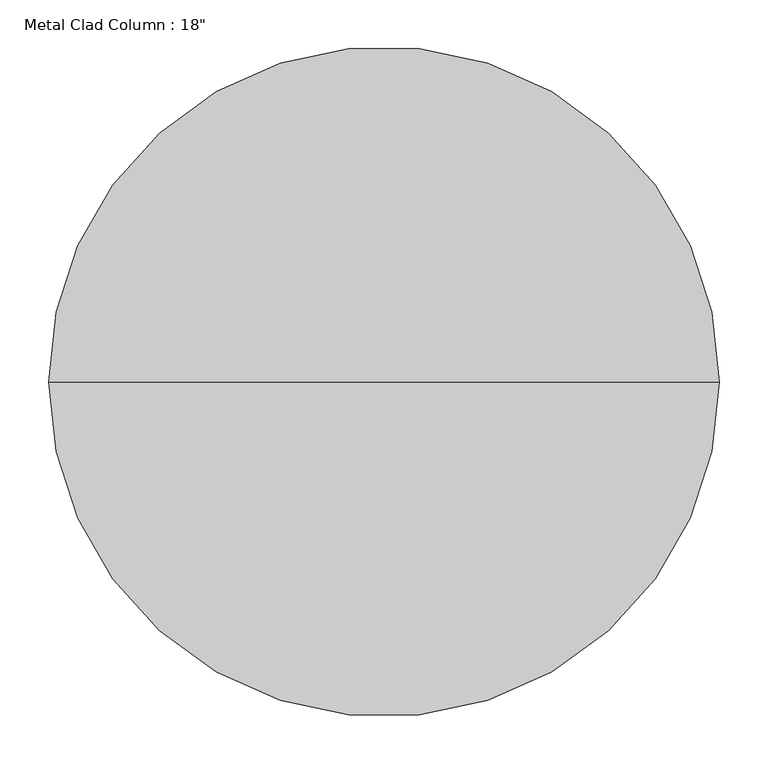
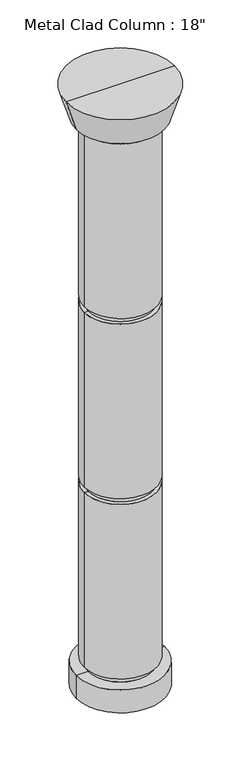
"""IFC4 building model written with IfcOpenShell, lengths in millimetres: column geometry."""

from ifc_helpers import new_model, si_unit, frame, origin, place, context, project, spatial, polyline, circle_curve, source, transform, mapped, element, save
from ifc_brep_helpers import plane_surface, cylinder_surface, revolved_surface, advanced_brep


def column_c029851a(model_context):
    return source(origin(), model_context, "Body", "AdvancedBrep", [
        advanced_brep(
        [(0.0, 0.0, 0.0), (-279.4, 0.0, 0.0), (279.4, 0.0, 0.0), (-279.4, 0.0, 152.4), (279.4, 0.0, 152.4), (203.2, 0.0, 1392.6), (-203.2, 0.0, 1392.6), (-228.6, 0.0, 1392.6), (228.6, 0.0, 1392.6), (-228.6, 0.0, 2556.6), (228.6, 0.0, 2556.6), (203.2, 0.0, 1354.5), (-203.2, 0.0, 1354.5), (228.6, 0.0, 1354.5), (-228.6, 0.0, 1354.5), (228.6, 0.0, 190.5), (-228.6, 0.0, 190.5), (203.2, 0.0, 190.5), (-203.2, 0.0, 190.5), (203.2, 0.0, 152.4), (-203.2, 0.0, 152.4), (279.4, 0.0, 3796.8), (-279.4, 0.0, 3796.8), (-342.9, 0.0, 4000.0), (342.9, 0.0, 4000.0), (0.0, 0.0, 4000.0), (203.2, 0.0, 3796.8), (-203.2, 0.0, 3796.8), (203.2, 0.0, 3758.7), (-203.2, 0.0, 3758.7), (228.6, 0.0, 3758.7), (-228.6, 0.0, 3758.7), (228.6, 0.0, 2594.7), (-228.6, 0.0, 2594.7), (203.2, 0.0, 2594.7), (-203.2, 0.0, 2594.7), (203.2, 0.0, 2556.6), (-203.2, 0.0, 2556.6)],
        [
            (0, 1),
            (1, 2, circle_curve(frame((0.0, 0.0, 0.0), z_axis=(0.0, 0.0, -1.0), x_axis=(-1.0, 0.0, 0.0)), 279.4)),
            (2, 0),
            (2, 1, circle_curve(frame((0.0, 0.0, 0.0), z_axis=(0.0, 0.0, -1.0), x_axis=(-1.0, 0.0, 0.0)), 279.4)),
            (1, 3),
            (3, 4, circle_curve(frame((0.0, 0.0, 152.4), z_axis=(0.0, 0.0, -1.0), x_axis=(-1.0, 0.0, 0.0)), 279.4)),
            (4, 2),
            (4, 3, circle_curve(frame((0.0, 0.0, 152.4), z_axis=(0.0, 0.0, -1.0), x_axis=(-1.0, 0.0, 0.0)), 279.4)),
            (5, 6, circle_curve(frame((0.0, 0.0, 1392.6), z_axis=(0.0, 0.0, 1.0), x_axis=(-1.0, 0.0, 0.0)), 203.2)),
            (6, 7),
            (7, 8, circle_curve(frame((0.0, 0.0, 1392.6), z_axis=(0.0, 0.0, -1.0), x_axis=(-1.0, 0.0, 0.0)), 228.6)),
            (8, 5),
            (7, 9),
            (9, 10, circle_curve(frame((0.0, 0.0, 2556.6), z_axis=(0.0, 0.0, -1.0), x_axis=(-1.0, 0.0, 0.0)), 228.6)),
            (10, 8),
            (7, 8, circle_curve(frame((0.0, 0.0, 1392.6), z_axis=(0.0, 0.0, 1.0), x_axis=(-1.0, 0.0, 0.0)), 228.6)),
            (10, 9, circle_curve(frame((0.0, 0.0, 2556.6), z_axis=(0.0, 0.0, -1.0), x_axis=(-1.0, 0.0, 0.0)), 228.6)),
            (6, 5, circle_curve(frame((0.0, 0.0, 1392.6), z_axis=(0.0, 0.0, 1.0), x_axis=(-1.0, 0.0, 0.0)), 203.2)),
            (11, 12, circle_curve(frame((0.0, 0.0, 1354.5), z_axis=(0.0, 0.0, 1.0), x_axis=(-1.0, 0.0, 0.0)), 203.2)),
            (12, 6),
            (5, 11),
            (12, 11, circle_curve(frame((0.0, 0.0, 1354.5), z_axis=(0.0, 0.0, 1.0), x_axis=(-1.0, 0.0, 0.0)), 203.2)),
            (13, 14, circle_curve(frame((0.0, 0.0, 1354.5), z_axis=(0.0, 0.0, 1.0), x_axis=(-1.0, 0.0, 0.0)), 228.6)),
            (14, 12),
            (11, 13),
            (14, 13, circle_curve(frame((0.0, 0.0, 1354.5), z_axis=(0.0, 0.0, 1.0), x_axis=(-1.0, 0.0, 0.0)), 228.6)),
            (15, 16, circle_curve(frame((0.0, 0.0, 190.5), z_axis=(0.0, 0.0, 1.0), x_axis=(-1.0, 0.0, 0.0)), 228.6)),
            (16, 14),
            (13, 15),
            (16, 15, circle_curve(frame((0.0, 0.0, 190.5), z_axis=(0.0, 0.0, 1.0), x_axis=(-1.0, 0.0, 0.0)), 228.6)),
            (17, 18, circle_curve(frame((0.0, 0.0, 190.5), z_axis=(0.0, 0.0, 1.0), x_axis=(-1.0, 0.0, 0.0)), 203.2)),
            (18, 16),
            (15, 17),
            (18, 17, circle_curve(frame((0.0, 0.0, 190.5), z_axis=(0.0, 0.0, 1.0), x_axis=(-1.0, 0.0, 0.0)), 203.2)),
            (19, 20, circle_curve(frame((0.0, 0.0, 152.4), z_axis=(0.0, 0.0, 1.0), x_axis=(-1.0, 0.0, 0.0)), 203.2)),
            (20, 18),
            (17, 19),
            (20, 19, circle_curve(frame((0.0, 0.0, 152.4), z_axis=(0.0, 0.0, 1.0), x_axis=(-1.0, 0.0, 0.0)), 203.2)),
            (3, 20),
            (19, 4),
            (21, 22, circle_curve(frame((0.0, 0.0, 3796.8), z_axis=(0.0, 0.0, 1.0), x_axis=(-1.0, 0.0, 0.0)), 279.4)),
            (22, 23),
            (23, 24, circle_curve(frame((0.0, 0.0, 4000.0), z_axis=(0.0, 0.0, -1.0), x_axis=(-1.0, 0.0, 0.0)), 342.9)),
            (24, 21),
            (23, 25),
            (25, 24),
            (23, 24, circle_curve(frame((0.0, 0.0, 4000.0), z_axis=(0.0, 0.0, 1.0), x_axis=(-1.0, 0.0, 0.0)), 342.9)),
            (22, 21, circle_curve(frame((0.0, 0.0, 3796.8), z_axis=(0.0, 0.0, 1.0), x_axis=(-1.0, 0.0, 0.0)), 279.4)),
            (26, 27, circle_curve(frame((0.0, 0.0, 3796.8), z_axis=(0.0, 0.0, 1.0), x_axis=(-1.0, 0.0, 0.0)), 203.2)),
            (27, 22),
            (21, 26),
            (27, 26, circle_curve(frame((0.0, 0.0, 3796.8), z_axis=(0.0, 0.0, 1.0), x_axis=(-1.0, 0.0, 0.0)), 203.2)),
            (28, 29, circle_curve(frame((0.0, 0.0, 3758.7), z_axis=(0.0, 0.0, 1.0), x_axis=(-1.0, 0.0, 0.0)), 203.2)),
            (29, 27),
            (26, 28),
            (29, 28, circle_curve(frame((0.0, 0.0, 3758.7), z_axis=(0.0, 0.0, 1.0), x_axis=(-1.0, 0.0, 0.0)), 203.2)),
            (30, 31, circle_curve(frame((0.0, 0.0, 3758.7), z_axis=(0.0, 0.0, 1.0), x_axis=(-1.0, 0.0, 0.0)), 228.6)),
            (31, 29),
            (28, 30),
            (31, 30, circle_curve(frame((0.0, 0.0, 3758.7), z_axis=(0.0, 0.0, 1.0), x_axis=(-1.0, 0.0, 0.0)), 228.6)),
            (32, 33, circle_curve(frame((0.0, 0.0, 2594.7), z_axis=(0.0, 0.0, 1.0), x_axis=(-1.0, 0.0, 0.0)), 228.6)),
            (33, 31),
            (30, 32),
            (33, 32, circle_curve(frame((0.0, 0.0, 2594.7), z_axis=(0.0, 0.0, 1.0), x_axis=(-1.0, 0.0, 0.0)), 228.6)),
            (34, 35, circle_curve(frame((0.0, 0.0, 2594.7), z_axis=(0.0, 0.0, 1.0), x_axis=(-1.0, 0.0, 0.0)), 203.2)),
            (35, 33),
            (32, 34),
            (35, 34, circle_curve(frame((0.0, 0.0, 2594.7), z_axis=(0.0, 0.0, 1.0), x_axis=(-1.0, 0.0, 0.0)), 203.2)),
            (36, 37, circle_curve(frame((0.0, 0.0, 2556.6), z_axis=(0.0, 0.0, 1.0), x_axis=(-1.0, 0.0, 0.0)), 203.2)),
            (37, 35),
            (34, 36),
            (37, 36, circle_curve(frame((0.0, 0.0, 2556.6), z_axis=(0.0, 0.0, 1.0), x_axis=(-1.0, 0.0, 0.0)), 203.2)),
            (9, 37),
            (36, 10),
        ],
        [
            plane_surface(frame((0.0, 0.0, 0.0), z_axis=(0.0, 0.0, -1.0), x_axis=(-1.0, 0.0, 0.0))),
            cylinder_surface(frame((0.0, 0.0, 4000.0), z_axis=(0.0, 0.0, -1.0), x_axis=(-1.0, 0.0, 0.0)), 279.4),
            plane_surface(frame((0.0, 0.0, 1392.6), z_axis=(0.0, 0.0, -1.0), x_axis=(-1.0, 0.0, 0.0))),
            cylinder_surface(frame((0.0, 0.0, 4000.0), z_axis=(0.0, 0.0, -1.0), x_axis=(-1.0, 0.0, 0.0)), 228.6),
            cylinder_surface(frame((0.0, 0.0, 4000.0), z_axis=(0.0, 0.0, -1.0), x_axis=(-1.0, 0.0, 0.0)), 203.2),
            plane_surface(frame((0.0, 0.0, 1354.5), z_axis=(0.0, 0.0, 1.0), x_axis=(-1.0, 0.0, 0.0))),
            plane_surface(frame((0.0, 0.0, 190.5), z_axis=(0.0, 0.0, -1.0), x_axis=(-1.0, 0.0, 0.0))),
            plane_surface(frame((0.0, 0.0, 152.4), z_axis=(0.0, 0.0, 1.0), x_axis=(-1.0, 0.0, 0.0))),
            revolved_surface(polyline([(-342.9, 0.0, 4000.0), (-279.4, 0.0, 3796.8)]), (0.0, 0.0, 4000.0), (0.0, 0.0, -1.0)),
            plane_surface(frame((0.0, 0.0, 4000.0), z_axis=(0.0, 0.0, 1.0), x_axis=(-1.0, 0.0, 0.0))),
            plane_surface(frame((0.0, 0.0, 3796.8), z_axis=(0.0, 0.0, -1.0), x_axis=(-1.0, 0.0, 0.0))),
            plane_surface(frame((0.0, 0.0, 3758.7), z_axis=(0.0, 0.0, 1.0), x_axis=(-1.0, 0.0, 0.0))),
            plane_surface(frame((0.0, 0.0, 2594.7), z_axis=(0.0, 0.0, -1.0), x_axis=(-1.0, 0.0, 0.0))),
            plane_surface(frame((0.0, 0.0, 2556.6), z_axis=(0.0, 0.0, 1.0), x_axis=(-1.0, 0.0, 0.0))),
        ],
        [
            (0, [[1, 2, 3]]),
            (0, [[-3, 4, -1]]),
            (1, [[-2, 5, 6, 7]]),
            (1, [[-4, -7, 8, -5]]),
            (2, [[9, 10, 11, 12]]),
            (3, [[-11, 13, 14, 15]]),
            (3, [[16, -15, 17, -13]]),
            (2, [[18, -12, -16, -10]]),
            (4, [[19, 20, -9, 21]]),
            (4, [[22, -21, -18, -20]]),
            (5, [[23, 24, -19, 25]]),
            (5, [[26, -25, -22, -24]]),
            (3, [[27, 28, -23, 29]]),
            (3, [[30, -29, -26, -28]]),
            (6, [[31, 32, -27, 33]]),
            (6, [[34, -33, -30, -32]]),
            (4, [[35, 36, -31, 37]]),
            (4, [[38, -37, -34, -36]]),
            (7, [[-6, 39, -35, 40]]),
            (7, [[-8, -40, -38, -39]]),
            (8, [[41, 42, 43, 44]]),
            (9, [[-43, 45, 46]]),
            (9, [[47, -46, -45]]),
            (8, [[48, -44, -47, -42]]),
            (10, [[49, 50, -41, 51]]),
            (10, [[52, -51, -48, -50]]),
            (4, [[53, 54, -49, 55]]),
            (4, [[56, -55, -52, -54]]),
            (11, [[57, 58, -53, 59]]),
            (11, [[60, -59, -56, -58]]),
            (3, [[61, 62, -57, 63]]),
            (3, [[64, -63, -60, -62]]),
            (12, [[65, 66, -61, 67]]),
            (12, [[68, -67, -64, -66]]),
            (4, [[69, 70, -65, 71]]),
            (4, [[72, -71, -68, -70]]),
            (13, [[-14, 73, -69, 74]]),
            (13, [[-17, -74, -72, -73]]),
        ],
    ),
    ])


if __name__ == "__main__":
    model = new_model("IFC4")
    model_context = context("Model", 3, world=origin())
    ifc_project = project(units=[si_unit("LENGTHUNIT", "METRE", prefix="MILLI")], contexts=[model_context])
    site = spatial("IfcSite", under=ifc_project)
    building = spatial("IfcBuilding", under=site)
    placement = place(None, origin())
    column_shape = column_c029851a(model_context)
    element("IfcColumn", 1, ObjectType="Metal Clad Column : 18\"", at=placement, inside=building, context=model_context, shape_type="MappedRepresentation", body=[
        mapped(column_shape, transform((0.0, 0.0, 0.0), x_axis=(1.0, 0.0, 0.0), y_axis=(0.0, 1.0, 0.0), z_axis=(0.0, 0.0, 1.0))),
    ])
    save(model, "model.ifc")

# Revit data of these elements
# Type "Metal Clad Column : 18\""
#   Assembly Code = "B1010200"
#   Base = 152.4 mm
#   Capital = 203.2 mm
#   Diameter = 457.2 mm
#   Joint Depth = 25.4 mm
#   Joint Width = 38.1 mm
#   Offset base level = 0 mm
#   Offset top level = 0 mm
#   Material = Aluminum
# Element 1 (IfcColumn, "Metal Clad Column : 18\"")
#   Materials on its faces: "Aluminum"
# Materials
#   "Aluminum": class "Metal", colour RGB 247 247 247, transparency 0, Description = "Aluminum 6061", Cost = 0
